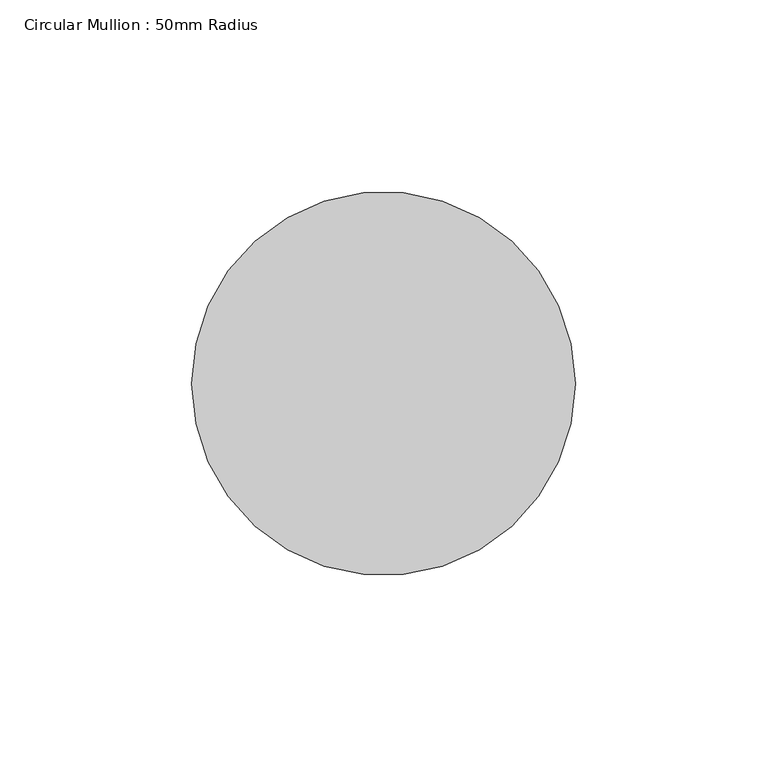
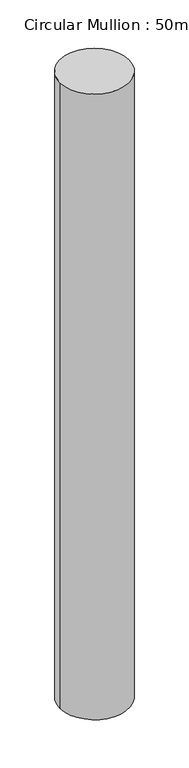
"""IFC4 building model written with IfcOpenShell, lengths in millimetres: member geometry, Circular Mullion : 50mm Radius."""

import ifcopenshell
import ifcopenshell.guid

model = None  # the IFC model being written
_history = None  # IfcOwnerHistory: only IFC2X3 demands one
_inside = {}  # id of a spatial element -> (the spatial element, [elements in it])
_under = {}  # id of a project, library or spatial element -> (it, [spatial elements below it])
_declared = {}  # id of a project -> (the project, [libraries it declares])
_typed = {}  # id of a type object -> (the type object, [elements of that type])
_made_of = {}  # id of a material, layer set ... -> (it, [elements and type objects made of it])


def new_model(schema):
    """Start an empty IFC model of exactly this schema.

    Asked for "IFC4X3", IfcOpenShell would pick the latest addendum, in which some entities
    have other attributes; the version numbers below select the first issue.
    IFC2X3 requires an IfcOwnerHistory on every rooted entity: one is made here for all.
    """
    global model, _history
    if schema == "IFC4X3":
        model = ifcopenshell.file(schema_version=(4, 3, 0, 0))
    else:
        model = ifcopenshell.file(schema=schema)
    _inside.clear()
    _under.clear()
    _declared.clear()
    _typed.clear()
    _made_of.clear()
    _history = None
    if model.schema == "IFC2X3":
        org = make("IfcOrganization", Name="unknown")
        user = make(
            "IfcPersonAndOrganization",
            ThePerson=make("IfcPerson", FamilyName="unknown"),
            TheOrganization=org,
        )
        app = make(
            "IfcApplication",
            ApplicationDeveloper=org,
            Version="unknown",
            ApplicationFullName="unknown",
            ApplicationIdentifier="unknown",
        )
        _history = make(
            "IfcOwnerHistory",
            OwningUser=user,
            OwningApplication=app,
            ChangeAction="ADDED",
            CreationDate=0,
        )
    return model


def make(cls, **values):
    """One entity of the class cls with the attributes given. An attribute that is None is left unset."""
    return model.create_entity(
        cls, **{name: value for name, value in values.items() if value is not None}
    )


def rooted(cls, **values):
    """An entity with a GlobalId (a new one), such as an element, a storey or a relation."""
    return make(cls, GlobalId=ifcopenshell.guid.new(), OwnerHistory=_history, **values)


def si_unit(unit_type, name, prefix=None):
    """IfcSIUnit, for example si_unit("LENGTHUNIT", "METRE", prefix="MILLI")."""
    return make("IfcSIUnit", UnitType=unit_type, Prefix=prefix, Name=name)


def assignment(units):
    """IfcUnitAssignment: the units of a project."""
    return None if units is None else make("IfcUnitAssignment", Units=units)


def point(xyz):
    """IfcCartesianPoint."""
    return None if xyz is None else make("IfcCartesianPoint", Coordinates=xyz)


def direction(xyz):
    """IfcDirection."""
    return None if xyz is None else make("IfcDirection", DirectionRatios=xyz)


def frame(location, z_axis=None, x_axis=None):
    """IfcAxis2Placement3D, a coordinate frame: its origin and axes. An axis left out is left unset."""
    return make(
        "IfcAxis2Placement3D",
        Location=point(location),
        Axis=direction(z_axis),
        RefDirection=direction(x_axis),
    )


def frame_2d(location, x_axis=None):
    """IfcAxis2Placement2D, a coordinate frame in the plane: its origin and x axis."""
    return make(
        "IfcAxis2Placement2D", Location=point(location), RefDirection=direction(x_axis)
    )


def origin():
    """The frame at (0, 0, 0) with its axes left unset."""
    return frame((0.0, 0.0, 0.0))


def origin_2d():
    """The frame at (0, 0) in the plane with its x axis left unset."""
    return frame_2d((0.0, 0.0))


def place(relative_to, where):
    """IfcLocalPlacement: puts the frame where relative to a parent placement (None: the world)."""
    return make(
        "IfcLocalPlacement", PlacementRelTo=relative_to, RelativePlacement=where
    )


def context(
    kind, dimensions, precision=None, world=None, true_north=None, identifier=None
):
    """IfcGeometricRepresentationContext, for example the 3D "Model" context."""
    return make(
        "IfcGeometricRepresentationContext",
        ContextIdentifier=identifier,
        ContextType=kind,
        CoordinateSpaceDimension=dimensions,
        Precision=precision,
        WorldCoordinateSystem=world,
        TrueNorth=true_north,
    )


def project(units=None, contexts=None):
    """IfcProject with its units and contexts."""
    return rooted(
        "IfcProject",
        Name="project",
        RepresentationContexts=contexts,
        UnitsInContext=assignment(units),
    )


def spatial(cls, under=None, at=None, **own):
    """A site, building, storey or space (cls), placed at a placement, below another one or the project."""
    s = rooted(cls, ObjectPlacement=at, **own)
    if under is not None:
        _under.setdefault(under.id(), (under, []))[1].append(s)
    return s


def circle_curve(where, radius):
    """IfcCircle in the frame where."""
    return make("IfcCircle", Position=where, Radius=radius)


def trimmed(basis, trim1, trim2, sense, master):
    """IfcTrimmedCurve: the piece of a basis curve between two trims."""
    return make(
        "IfcTrimmedCurve",
        BasisCurve=basis,
        Trim1=trim1,
        Trim2=trim2,
        SenseAgreement=sense,
        MasterRepresentation=master,
    )


def segment(curve, same_sense, transition):
    """IfcCompositeCurveSegment."""
    return make(
        "IfcCompositeCurveSegment",
        Transition=transition,
        SameSense=same_sense,
        ParentCurve=curve,
    )


def composite_curve(segments, self_intersect=None):
    """IfcCompositeCurve: segments joined end to end."""
    return make("IfcCompositeCurve", Segments=segments, SelfIntersect=self_intersect)


def outline(outer, holes=None, kind="AREA"):
    """IfcArbitraryClosedProfileDef: a profile drawn as a closed curve; with holes, ...WithVoids."""
    if holes is None:
        return make("IfcArbitraryClosedProfileDef", ProfileType=kind, OuterCurve=outer)
    return make(
        "IfcArbitraryProfileDefWithVoids",
        ProfileType=kind,
        OuterCurve=outer,
        InnerCurves=holes,
    )


def extrude(swept, where, along, depth):
    """IfcExtrudedAreaSolid: the profile swept, set in the frame where, extruded along a direction by depth."""
    return make(
        "IfcExtrudedAreaSolid",
        SweptArea=swept,
        Position=where,
        ExtrudedDirection=direction(along),
        Depth=depth,
    )


def shape(context_of_items, identifier, shape_type, items):
    """IfcShapeRepresentation: the items that make up one representation, for example the "Body"."""
    return make(
        "IfcShapeRepresentation",
        ContextOfItems=context_of_items,
        RepresentationIdentifier=identifier,
        RepresentationType=shape_type,
        Items=items,
    )


def source(mapping_origin, context_of_items, identifier, shape_type, items):
    """IfcRepresentationMap: a shape defined once, which mapped items show again and again."""
    return make(
        "IfcRepresentationMap",
        MappingOrigin=mapping_origin,
        MappedRepresentation=shape(context_of_items, identifier, shape_type, items),
    )


def transform(
    local_origin,
    x_axis=None,
    y_axis=None,
    z_axis=None,
    scale=None,
    scale2=None,
    scale3=None,
    uniform=True,
):
    """IfcCartesianTransformationOperator3D, or its non-uniform kind. x_axis, y_axis, z_axis: its Axis1, 2, 3."""
    if uniform:
        return make(
            "IfcCartesianTransformationOperator3D",
            Axis1=direction(x_axis),
            Axis2=direction(y_axis),
            LocalOrigin=point(local_origin),
            Scale=scale,
            Axis3=direction(z_axis),
        )
    return make(
        "IfcCartesianTransformationOperator3DnonUniform",
        Axis1=direction(x_axis),
        Axis2=direction(y_axis),
        LocalOrigin=point(local_origin),
        Scale=scale,
        Axis3=direction(z_axis),
        Scale2=scale2,
        Scale3=scale3,
    )


def mapped(mapping_source, mapping_target):
    """IfcMappedItem: shows the shape of a source again, moved by a transform."""
    return make(
        "IfcMappedItem", MappingSource=mapping_source, MappingTarget=mapping_target
    )


def made_of(thing, what):
    """Note that an element or type object is made of a material, layer set ...; save() writes the relation."""
    if what is not None:
        _made_of.setdefault(what.id(), (what, []))[1].append(thing)
    return thing


def element(
    cls,
    number,
    at=None,
    inside=None,
    cuts=None,
    type_object=None,
    material=None,
    context=None,
    identifier="Body",
    shape_type=None,
    held_by="IfcProductDefinitionShape",
    body=None,
    shapes=None,
    **own,
):
    """One element of the class cls, such as IfcWall. Its Tag is "e" and its number.

    at: its placement. inside: the storey or other place that contains it. cuts: it is an
    opening in that element (IfcRelVoidsElement). A single representation is given by context,
    identifier, shape_type and body (its items); several are given by shapes. held_by: the class
    of the entity that holds the representations. save() writes the other relations.
    """
    e = rooted(cls, Tag="e%d" % number, ObjectPlacement=at, **own)
    if body is not None:
        shapes = [shape(context, identifier, shape_type, body)]
    if shapes is not None:
        e.Representation = make(held_by, Representations=shapes)
    if inside is not None:
        _inside.setdefault(inside.id(), (inside, []))[1].append(e)
    if cuts is not None:
        rooted(
            "IfcRelVoidsElement", RelatingBuildingElement=cuts, RelatedOpeningElement=e
        )
    if type_object is not None:
        _typed.setdefault(type_object.id(), (type_object, []))[1].append(e)
    return made_of(e, material)


def aggregate(whole, parts):
    """IfcRelAggregates: a whole, such as a stair, and the parts it consists of."""
    return rooted("IfcRelAggregates", RelatingObject=whole, RelatedObjects=parts)


def save(model, path):
    """Write the relations noted so far, then the file.

    IfcRelAggregates (storeys below a building ...), IfcRelContainedInSpatialStructure (elements
    in a storey), IfcRelDefinesByType, IfcRelAssociatesMaterial and IfcRelDeclares: one each for
    every whole, place, type object, material and project.
    """
    for whole, parts in _under.values():
        aggregate(whole, parts)
    for where, things in _inside.values():
        rooted(
            "IfcRelContainedInSpatialStructure",
            RelatedElements=things,
            RelatingStructure=where,
        )
    for kind, things in _typed.values():
        rooted("IfcRelDefinesByType", RelatedObjects=things, RelatingType=kind)
    for what, things in _made_of.values():
        rooted("IfcRelAssociatesMaterial", RelatedObjects=things, RelatingMaterial=what)
    for by, libraries in _declared.values():
        rooted("IfcRelDeclares", RelatingContext=by, RelatedDefinitions=libraries)
    model.write(path)


def circular_mullion_50mm_radius_f2d53690(model_context):
    return source(origin(), model_context, "Body", "SweptSolid", [
        extrude(outline(composite_curve([segment(trimmed(circle_curve(origin_2d(), 50.0), [point((50.0, 0.0))], [point((-50.0, 0.0))], False, "CARTESIAN"), True, "CONTINUOUS"), segment(trimmed(circle_curve(origin_2d(), 50.0), [point((-50.0, 0.0))], [point((50.0, 0.0))], False, "CARTESIAN"), True, "CONTINUOUS")], self_intersect=False)), frame((0.0, 0.0, -957.7497981), z_axis=(0.0, 0.0, 1.0), x_axis=(1.0, 0.0, 0.0)), (0.0, 0.0, 1.0), 957.7497981),
    ])


if __name__ == "__main__":
    model = new_model("IFC4")
    model_context = context("Model", 3, world=origin())
    ifc_project = project(units=[si_unit("LENGTHUNIT", "METRE", prefix="MILLI")], contexts=[model_context])
    site = spatial("IfcSite", under=ifc_project)
    building = spatial("IfcBuilding", under=site)
    placement = place(None, origin())
    circular_mullion_50mm_radius_shape = circular_mullion_50mm_radius_f2d53690(model_context)
    element("IfcMember", 1, ObjectType="Circular Mullion : 50mm Radius", at=placement, inside=building, context=model_context, shape_type="MappedRepresentation", body=[
        mapped(circular_mullion_50mm_radius_shape, transform((0.0, 0.0, 0.0), x_axis=(1.0, 0.0, 0.0), y_axis=(0.0, 1.0, 0.0), z_axis=(0.0, 0.0, 1.0))),
    ])
    save(model, "model.ifc")

# Revit data of these elements
# Type "Circular Mullion : 50mm Radius"
#   built-in parameter 1007350 = 0.164042 (stored number, unit not read)
# Element 1 (IfcMember, "Circular Mullion : 50mm Radius")
#   Materials on its faces: "Aluminium"
# Materials
#   "Aluminium": class "Metal", colour RGB 247 247 247, transparency 0, Description = "Aluminium 6061", Cost = 0
